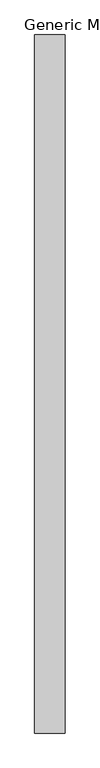
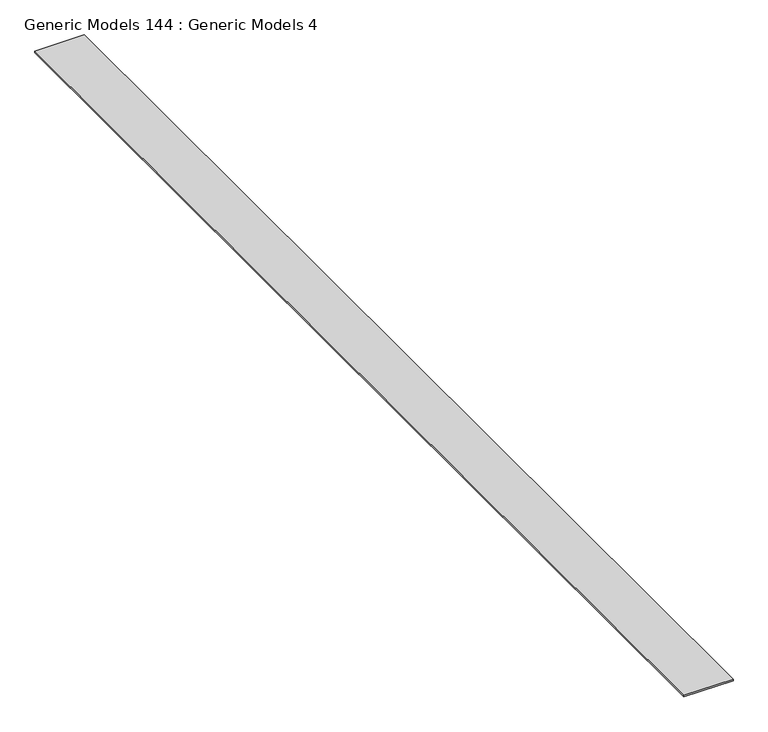
"""IFC4 building model written with IfcOpenShell, lengths in millimetres: proxy geometry, Generic Models 144 : Generic Models 4."""

from ifc_helpers import new_model, si_unit, frame, origin, place, context, project, spatial, polyline, outline, extrude, source, transform, mapped, element, save


def generic_models_144_generic_models_4_4e374bbd(model_context):
    return source(origin(), model_context, "Body", "SweptSolid", [
        extrude(outline(polyline([(-5950.1236296, -5493.3230338), (-6498.6122941, -5493.3230338), (-6498.6122941, 7054.2769662), (-5950.1236296, 7054.2769662), (-5950.1236296, -5493.3230338)])), frame((0.0, 0.0, 123261.1835), z_axis=(0.0, 0.0, 1.0), x_axis=(1.0, 0.0, 0.0)), (0.0, 0.0, 1.0), 17.4625),
    ])


if __name__ == "__main__":
    model = new_model("IFC4")
    model_context = context("Model", 3, world=origin())
    ifc_project = project(units=[si_unit("LENGTHUNIT", "METRE", prefix="MILLI")], contexts=[model_context])
    site = spatial("IfcSite", under=ifc_project)
    building = spatial("IfcBuilding", under=site)
    placement = place(None, origin())
    generic_models_144_generic_models_4_shape = generic_models_144_generic_models_4_4e374bbd(model_context)
    element("IfcBuildingElementProxy", 1, Name="Generic Models 144 : Generic Models 4", ObjectType="Generic Models 144 : Generic Models 4", at=placement, inside=building, context=model_context, shape_type="MappedRepresentation", body=[
        mapped(generic_models_144_generic_models_4_shape, transform((0.0, 0.0, 0.0), x_axis=(1.0, 0.0, 0.0), y_axis=(0.0, 1.0, 0.0), z_axis=(0.0, 0.0, 1.0))),
    ])
    save(model, "model.ifc")

# Revit data of these elements
# Element 1 (IfcBuildingElementProxy, "Generic Models 144 : Generic Models 4")
#   Materials on its faces: "_CDX PLYWOOD -  SEE STRUCT DWGs"
# Materials
#   "_CDX PLYWOOD -  SEE STRUCT DWGs": class "Generic", colour RGB 98 75 74, transparency 0, Cost = 0
